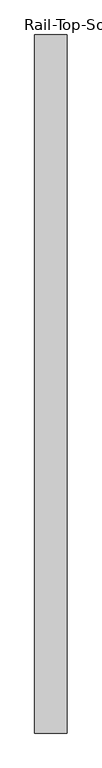
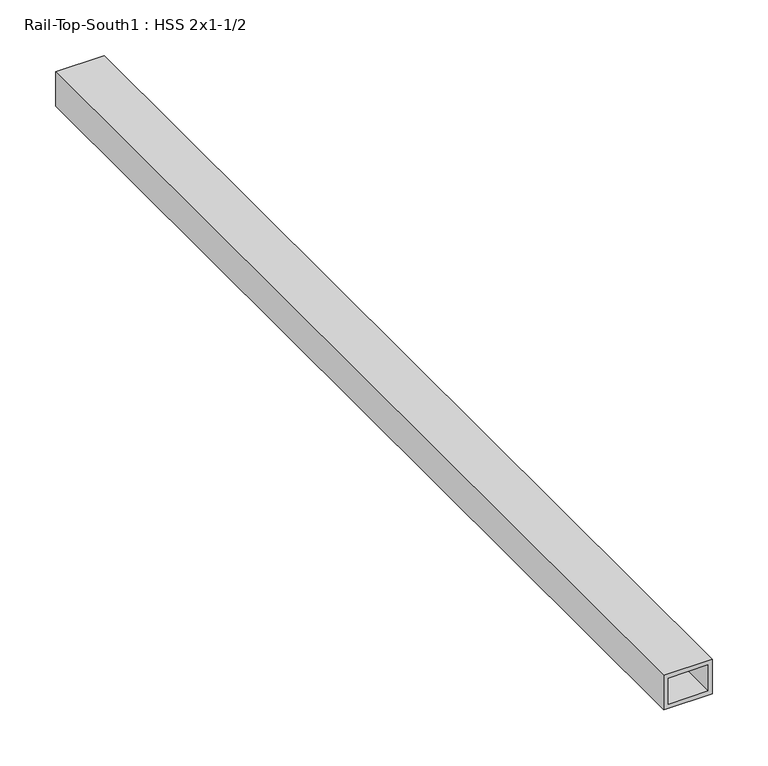
"""IFC4 building model written with IfcOpenShell, lengths in millimetres: proxy geometry, Rail-Top-South1 : HSS 2x1-1/2."""

from ifc_helpers import new_model, si_unit, frame, origin, place, context, project, spatial, polyline, outline, extrude, source, transform, mapped, element, save


def rail_top_south1_hss_2x1_1_2_6b80f164(model_context):
    return source(origin(), model_context, "Body", "SweptSolid", [
        extrude(outline(polyline([(2400.3, 587416.6934739), (2438.4, 587416.6934739), (2438.4, 587365.8934739), (2400.3, 587365.8934739), (2400.3, 587416.6934739)]), holes=[polyline([(2433.6375, 587411.9309739), (2405.0625, 587411.9309739), (2405.0625, 587370.6559739), (2433.6375, 587370.6559739), (2433.6375, 587411.9309739)])]), frame((0.0, -536301.7038841, 0.0), z_axis=(0.0, 1.0, 0.0), x_axis=(0.0, 0.0, 1.0)), (0.0, 0.0, 1.0), 1093.7875),
    ])


if __name__ == "__main__":
    model = new_model("IFC4")
    model_context = context("Model", 3, world=origin())
    ifc_project = project(units=[si_unit("LENGTHUNIT", "METRE", prefix="MILLI")], contexts=[model_context])
    site = spatial("IfcSite", under=ifc_project)
    building = spatial("IfcBuilding", under=site)
    placement = place(None, origin())
    rail_top_south1_hss_2x1_1_2_shape = rail_top_south1_hss_2x1_1_2_6b80f164(model_context)
    element("IfcBuildingElementProxy", 1, Name="Rail-Top-South1 : HSS 2x1-1/2", ObjectType="Rail-Top-South1 : HSS 2x1-1/2", at=placement, inside=building, context=model_context, shape_type="MappedRepresentation", body=[
        mapped(rail_top_south1_hss_2x1_1_2_shape, transform((0.0, 0.0, 0.0), x_axis=(1.0, 0.0, 0.0), y_axis=(0.0, 1.0, 0.0), z_axis=(0.0, 0.0, 1.0))),
    ])
    save(model, "model.ifc")

# Revit data of these elements
# Element 1 (IfcBuildingElementProxy, "Rail-Top-South1 : HSS 2x1-1/2")
#   Materials on its faces: "1-1/2\"X2\" GALV. STL HSS TUBING"
# Materials
#   "1-1/2\"X2\" GALV. STL HSS TUBING": class "Generic", colour RGB 211 211 207, transparency 0, Cost = 0
